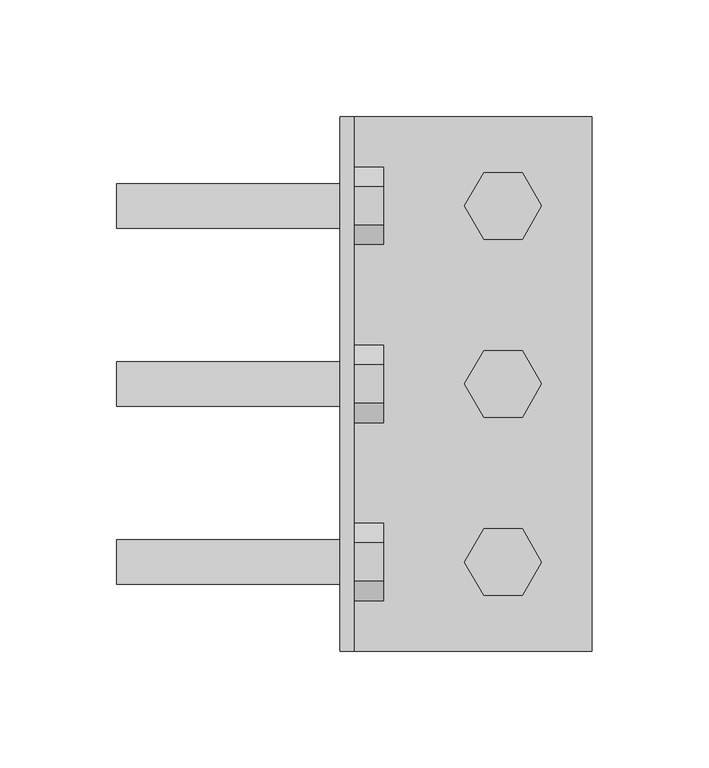
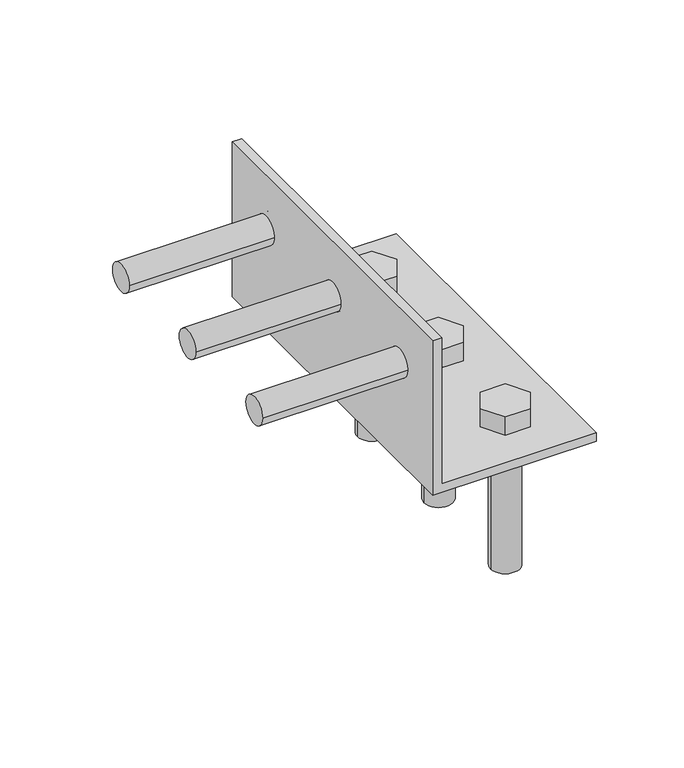
"""IFC4 building model written with IfcOpenShell, lengths in millimetres: fastener geometry, SIMPSON - HLPC/HLGPC Heavy Angles and Gussets : SIMPSON -HL49 - 9 X 4.25 - .75 Bolt - HDG."""

from ifc_helpers import new_model, si_unit, point, frame, frame_2d, origin, place, context, project, spatial, polyline, circle_curve, trimmed, segment, composite_curve, outline, extrude, source, transform, mapped, element, save
from ifc_brep_helpers import plane_surface, revolved_surface, advanced_brep


def fastener_80b0e17a(model_context):
    return source(origin(), model_context, "Body", "SolidModel", [
        extrude(outline(composite_curve([segment(trimmed(circle_curve(frame_2d((76.2, 69.85)), 9.525), [point((85.725, 69.85))], [point((66.675, 69.85))], False, "CARTESIAN"), True, "CONTINUOUS"), segment(trimmed(circle_curve(frame_2d((76.2, 69.85)), 9.525), [point((66.675, 69.85))], [point((85.725, 69.85))], False, "CARTESIAN"), True, "CONTINUOUS")], self_intersect=False)), frame((-95.5476562, 0.0, 0.0), z_axis=(1.0, 0.0, 0.0), x_axis=(0.0, 1.0, 0.0)), (0.0, 0.0, 1.0), 101.6),
        extrude(outline(polyline([(92.6977839, 69.85), (84.448892, 55.5625), (67.951108, 55.5625), (59.7022161, 69.85), (67.951108, 84.1375), (84.448892, 84.1375), (92.6977839, 69.85)])), frame((6.0523438, 0.0, 0.0), z_axis=(1.0, 0.0, 0.0), x_axis=(0.0, 1.0, 0.0)), (0.0, 0.0, 1.0), 12.7),
        extrude(outline(composite_curve([segment(trimmed(circle_curve(frame_2d((0.0, 69.85)), 9.525), [point((9.525, 69.85))], [point((-9.525, 69.85))], False, "CARTESIAN"), True, "CONTINUOUS"), segment(trimmed(circle_curve(frame_2d((0.0, 69.85)), 9.525), [point((-9.525, 69.85))], [point((9.525, 69.85))], False, "CARTESIAN"), True, "CONTINUOUS")], self_intersect=False)), frame((-95.5476562, 0.0, 0.0), z_axis=(1.0, 0.0, 0.0), x_axis=(0.0, 1.0, 0.0)), (0.0, 0.0, 1.0), 101.6),
        extrude(outline(polyline([(16.4977839, 69.85), (8.248892, 55.5625), (-8.248892, 55.5625), (-16.4977839, 69.85), (-8.248892, 84.1375), (8.248892, 84.1375), (16.4977839, 69.85)])), frame((6.0523438, 0.0, 0.0), z_axis=(1.0, 0.0, 0.0), x_axis=(0.0, 1.0, 0.0)), (0.0, 0.0, 1.0), 12.7),
        extrude(outline(composite_curve([segment(trimmed(circle_curve(frame_2d((-76.2, 69.85)), 9.525), [point((-66.675, 69.85))], [point((-85.725, 69.85))], False, "CARTESIAN"), True, "CONTINUOUS"), segment(trimmed(circle_curve(frame_2d((-76.2, 69.85)), 9.525), [point((-85.725, 69.85))], [point((-66.675, 69.85))], False, "CARTESIAN"), True, "CONTINUOUS")], self_intersect=False)), frame((-95.5476562, 0.0, 0.0), z_axis=(1.0, 0.0, 0.0), x_axis=(0.0, 1.0, 0.0)), (0.0, 0.0, 1.0), 101.6),
        extrude(outline(polyline([(-59.7022161, 69.85), (-67.951108, 55.5625), (-84.448892, 55.5625), (-92.6977839, 69.85), (-84.448892, 84.1375), (-67.951108, 84.1375), (-59.7022161, 69.85)])), frame((6.0523438, 0.0, 0.0), z_axis=(1.0, 0.0, 0.0), x_axis=(0.0, 1.0, 0.0)), (0.0, 0.0, 1.0), 12.7),
        extrude(outline(composite_curve([segment(trimmed(circle_curve(frame_2d((69.85, -76.2)), 9.525), [point((60.325, -76.2))], [point((79.375, -76.2))], False, "CARTESIAN"), True, "CONTINUOUS"), segment(trimmed(circle_curve(frame_2d((69.85, -76.2)), 9.525), [point((79.375, -76.2))], [point((60.325, -76.2))], False, "CARTESIAN"), True, "CONTINUOUS")], self_intersect=False)), frame((0.0, 0.0, -95.5476563), z_axis=(0.0, 0.0, 1.0), x_axis=(1.0, 0.0, 0.0)), (0.0, 0.0, 1.0), 101.6),
        extrude(outline(polyline([(53.3522161, -76.2), (61.601108, -61.9125), (78.098892, -61.9125), (86.3477839, -76.2), (78.098892, -90.4875), (61.601108, -90.4875), (53.3522161, -76.2)])), frame((0.0, 0.0, 6.0523437), z_axis=(0.0, 0.0, 1.0), x_axis=(1.0, 0.0, 0.0)), (0.0, 0.0, 1.0), 12.7),
        extrude(outline(composite_curve([segment(trimmed(circle_curve(frame_2d((69.85, 0.0)), 9.525), [point((60.325, 0.0))], [point((79.375, 0.0))], False, "CARTESIAN"), True, "CONTINUOUS"), segment(trimmed(circle_curve(frame_2d((69.85, 0.0)), 9.525), [point((79.375, 0.0))], [point((60.325, 0.0))], False, "CARTESIAN"), True, "CONTINUOUS")], self_intersect=False)), frame((0.0, 0.0, -95.5476563), z_axis=(0.0, 0.0, 1.0), x_axis=(1.0, 0.0, 0.0)), (0.0, 0.0, 1.0), 101.6),
        extrude(outline(polyline([(53.3522161, 0.0), (61.601108, 14.2875), (78.098892, 14.2875), (86.3477839, 0.0), (78.098892, -14.2875), (61.601108, -14.2875), (53.3522161, 0.0)])), frame((0.0, 0.0, 6.0523437), z_axis=(0.0, 0.0, 1.0), x_axis=(1.0, 0.0, 0.0)), (0.0, 0.0, 1.0), 12.7),
        extrude(outline(composite_curve([segment(trimmed(circle_curve(frame_2d((69.85, 76.2)), 9.525), [point((60.325, 76.2))], [point((79.375, 76.2))], False, "CARTESIAN"), True, "CONTINUOUS"), segment(trimmed(circle_curve(frame_2d((69.85, 76.2)), 9.525), [point((79.375, 76.2))], [point((60.325, 76.2))], False, "CARTESIAN"), True, "CONTINUOUS")], self_intersect=False)), frame((0.0, 0.0, -95.5476563), z_axis=(0.0, 0.0, 1.0), x_axis=(1.0, 0.0, 0.0)), (0.0, 0.0, 1.0), 101.6),
        extrude(outline(polyline([(53.3522161, 76.2), (61.601108, 90.4875), (78.098892, 90.4875), (86.3477839, 76.2), (78.098892, 61.9125), (61.601108, 61.9125), (53.3522161, 76.2)])), frame((0.0, 0.0, 6.0523437), z_axis=(0.0, 0.0, 1.0), x_axis=(1.0, 0.0, 0.0)), (0.0, 0.0, 1.0), 12.7),
        advanced_brep(
        [(6.0523438, -114.3, 107.95), (6.0523438, -114.3, 6.0523437), (6.0523438, 114.3, 6.0523437), (6.0523438, 114.3, 107.95), (6.0523438, 66.675, 69.85), (6.0523438, 85.725, 69.85), (6.0523438, -9.525, 69.85), (6.0523438, 9.525, 69.85), (6.0523438, -85.725, 69.85), (6.0523438, -66.675, 69.85), (0.0, 114.3, 107.95), (0.0, 114.3, 0.0), (0.0, -114.3, 0.0), (0.0, -114.3, 107.95), (0.0, 85.725, 69.85), (0.0, 66.675, 69.85), (0.0, 9.525, 69.85), (0.0, -9.525, 69.85), (0.0, -66.675, 69.85), (0.0, -85.725, 69.85), (107.95, 114.3, 6.0523437), (107.95, 114.3, 0.0), (107.95, -114.3, 0.0), (107.95, -114.3, 6.0523437), (79.375, 76.2, 6.0523437), (60.325, 76.2, 6.0523437), (79.375, 0.0, 6.0523437), (60.325, 0.0, 6.0523437), (79.375, -76.2, 6.0523437), (60.325, -76.2, 6.0523437), (60.325, 76.2, 0.0), (79.375, 76.2, 0.0), (60.325, 0.0, 0.0), (79.375, 0.0, 0.0), (60.325, -76.2, 0.0), (79.375, -76.2, 0.0)],
        [
            (0, 1),
            (1, 2),
            (2, 3),
            (3, 0),
            (4, 5, circle_curve(frame((6.0523438, 76.2, 69.85), z_axis=(-1.0, 0.0, 0.0), x_axis=(0.0, -1.0, 0.0)), 9.525)),
            (5, 4, circle_curve(frame((6.0523438, 76.2, 69.85), z_axis=(-1.0, 0.0, 0.0), x_axis=(0.0, -1.0, 0.0)), 9.525)),
            (6, 7, circle_curve(frame((6.0523438, 0.0, 69.85), z_axis=(-1.0, 0.0, 0.0), x_axis=(0.0, -1.0, 0.0)), 9.525)),
            (7, 6, circle_curve(frame((6.0523438, 0.0, 69.85), z_axis=(-1.0, 0.0, 0.0), x_axis=(0.0, -1.0, 0.0)), 9.525)),
            (8, 9, circle_curve(frame((6.0523438, -76.2, 69.85), z_axis=(-1.0, 0.0, 0.0), x_axis=(0.0, -1.0, 0.0)), 9.525)),
            (9, 8, circle_curve(frame((6.0523438, -76.2, 69.85), z_axis=(-1.0, 0.0, 0.0), x_axis=(0.0, -1.0, 0.0)), 9.525)),
            (10, 11),
            (11, 12),
            (12, 13),
            (13, 10),
            (14, 15, circle_curve(frame((0.0, 76.2, 69.85), z_axis=(1.0, 0.0, 0.0), x_axis=(0.0, -1.0, 0.0)), 9.525)),
            (15, 14, circle_curve(frame((0.0, 76.2, 69.85), z_axis=(1.0, 0.0, 0.0), x_axis=(0.0, -1.0, 0.0)), 9.525)),
            (16, 17, circle_curve(frame((0.0, 0.0, 69.85), z_axis=(1.0, 0.0, 0.0), x_axis=(0.0, -1.0, 0.0)), 9.525)),
            (17, 16, circle_curve(frame((0.0, 0.0, 69.85), z_axis=(1.0, 0.0, 0.0), x_axis=(0.0, -1.0, 0.0)), 9.525)),
            (18, 19, circle_curve(frame((0.0, -76.2, 69.85), z_axis=(1.0, 0.0, 0.0), x_axis=(0.0, -1.0, 0.0)), 9.525)),
            (19, 18, circle_curve(frame((0.0, -76.2, 69.85), z_axis=(1.0, 0.0, 0.0), x_axis=(0.0, -1.0, 0.0)), 9.525)),
            (3, 10),
            (13, 0),
            (2, 20),
            (20, 21),
            (21, 11),
            (12, 22),
            (22, 23),
            (23, 1),
            (23, 20),
            (24, 25, circle_curve(frame((69.85, 76.2, 6.0523437), z_axis=(0.0, 0.0, -1.0), x_axis=(1.0, 0.0, 0.0)), 9.525)),
            (25, 24, circle_curve(frame((69.85, 76.2, 6.0523437), z_axis=(0.0, 0.0, -1.0), x_axis=(1.0, 0.0, 0.0)), 9.525)),
            (26, 27, circle_curve(frame((69.85, 0.0, 6.0523437), z_axis=(0.0, 0.0, -1.0), x_axis=(1.0, 0.0, 0.0)), 9.525)),
            (27, 26, circle_curve(frame((69.85, 0.0, 6.0523437), z_axis=(0.0, 0.0, -1.0), x_axis=(1.0, 0.0, 0.0)), 9.525)),
            (28, 29, circle_curve(frame((69.85, -76.2, 6.0523437), z_axis=(0.0, 0.0, -1.0), x_axis=(1.0, 0.0, 0.0)), 9.525)),
            (29, 28, circle_curve(frame((69.85, -76.2, 6.0523437), z_axis=(0.0, 0.0, -1.0), x_axis=(1.0, 0.0, 0.0)), 9.525)),
            (21, 22),
            (30, 31, circle_curve(frame((69.85, 76.2, 0.0), z_axis=(0.0, 0.0, 1.0), x_axis=(1.0, 0.0, 0.0)), 9.525)),
            (31, 30, circle_curve(frame((69.85, 76.2, 0.0), z_axis=(0.0, 0.0, 1.0), x_axis=(1.0, 0.0, 0.0)), 9.525)),
            (32, 33, circle_curve(frame((69.85, 0.0, 0.0), z_axis=(0.0, 0.0, 1.0), x_axis=(1.0, 0.0, 0.0)), 9.525)),
            (33, 32, circle_curve(frame((69.85, 0.0, 0.0), z_axis=(0.0, 0.0, 1.0), x_axis=(1.0, 0.0, 0.0)), 9.525)),
            (34, 35, circle_curve(frame((69.85, -76.2, 0.0), z_axis=(0.0, 0.0, 1.0), x_axis=(1.0, 0.0, 0.0)), 9.525)),
            (35, 34, circle_curve(frame((69.85, -76.2, 0.0), z_axis=(0.0, 0.0, 1.0), x_axis=(1.0, 0.0, 0.0)), 9.525)),
            (25, 30),
            (31, 24),
            (27, 32),
            (33, 26),
            (29, 34),
            (35, 28),
            (5, 14),
            (15, 4),
            (7, 16),
            (17, 6),
            (9, 18),
            (19, 8),
        ],
        [
            plane_surface(frame((6.0523438, 114.3, 107.95), z_axis=(1.0, 0.0, 0.0), x_axis=(0.0, 1.0, 0.0))),
            plane_surface(frame((0.0, 114.3, 107.95), z_axis=(-1.0, 0.0, 0.0), x_axis=(0.0, -1.0, 0.0))),
            plane_surface(frame((6.0523438, -114.3, 107.95), z_axis=(0.0, 0.0, 1.0), x_axis=(-1.0, 0.0, 0.0))),
            plane_surface(frame((6.0523438, 114.3, 107.95), z_axis=(0.0, 1.0, 0.0), x_axis=(-1.0, 0.0, 0.0))),
            plane_surface(frame((6.0523438, -114.3, 6.0523437), z_axis=(0.0, -1.0, 0.0), x_axis=(-1.0, 0.0, 0.0))),
            plane_surface(frame((0.0, -114.3, 6.0523437), z_axis=(0.0, 0.0, 1.0), x_axis=(-1.0, 0.0, 0.0))),
            plane_surface(frame((0.0, -114.3, 0.0), z_axis=(0.0, 0.0, -1.0), x_axis=(1.0, 0.0, 0.0))),
            plane_surface(frame((107.95, 114.3, 6.0523437), z_axis=(1.0, 0.0, 0.0), x_axis=(0.0, 0.0, -1.0))),
            revolved_surface(polyline([(79.375, 76.2, 6.0523437), (79.375, 76.2, 0.0)]), (69.85, 76.2, 0.0), (0.0, 0.0, 1.0)),
            revolved_surface(polyline([(79.375, 0.0, 6.0523437), (79.375, 0.0, 0.0)]), (69.85, 0.0, 0.0), (0.0, 0.0, 1.0)),
            revolved_surface(polyline([(79.375, -76.2, 6.0523437), (79.375, -76.2, 0.0)]), (69.85, -76.2, 0.0), (0.0, 0.0, 1.0)),
            revolved_surface(polyline([(6.0523438, 66.675, 69.85), (0.0, 66.675, 69.85)]), (0.0, 76.2, 69.85), (1.0, 0.0, 0.0)),
            revolved_surface(polyline([(6.0523438, -9.525, 69.85), (0.0, -9.525, 69.85)]), (0.0, 0.0, 69.85), (1.0, 0.0, 0.0)),
            revolved_surface(polyline([(6.0523438, -85.72500000000001, 69.85), (0.0, -85.72500000000001, 69.85)]), (0.0, -76.2, 69.85), (1.0, 0.0, 0.0)),
        ],
        [
            (0, [[1, 2, 3, 4], [5, 6], [7, 8], [9, 10]]),
            (1, [[11, 12, 13, 14], [15, 16], [17, 18], [19, 20]]),
            (2, [[21, -14, 22, -4]]),
            (3, [[23, 24, 25, -11, -21, -3]]),
            (4, [[-22, -13, 26, 27, 28, -1]]),
            (5, [[-23, -2, -28, 29], [30, 31], [32, 33], [34, 35]]),
            (6, [[-26, -12, -25, 36], [37, 38], [39, 40], [41, 42]]),
            (7, [[-27, -36, -24, -29]]),
            (8, [[-31, 43, -38, 44]]),
            (8, [[-37, -43, -30, -44]]),
            (9, [[-33, 45, -40, 46]]),
            (9, [[-39, -45, -32, -46]]),
            (10, [[-35, 47, -42, 48]]),
            (10, [[-41, -47, -34, -48]]),
            (11, [[-6, 49, -16, 50]]),
            (11, [[-15, -49, -5, -50]]),
            (12, [[-8, 51, -18, 52]]),
            (12, [[-17, -51, -7, -52]]),
            (13, [[-10, 53, -20, 54]]),
            (13, [[-19, -53, -9, -54]]),
        ],
    ),
    ])


if __name__ == "__main__":
    model = new_model("IFC4")
    model_context = context("Model", 3, world=origin())
    ifc_project = project(units=[si_unit("LENGTHUNIT", "METRE", prefix="MILLI")], contexts=[model_context])
    site = spatial("IfcSite", under=ifc_project)
    building = spatial("IfcBuilding", under=site)
    placement = place(None, origin())
    fastener_shape = fastener_80b0e17a(model_context)
    element("IfcFastener", 1, ObjectType="SIMPSON - HLPC/HLGPC Heavy Angles and Gussets : SIMPSON -HL49 - 9 X 4.25 - .75 Bolt - HDG", at=placement, inside=building, context=model_context, shape_type="MappedRepresentation", body=[
        mapped(fastener_shape, transform((0.0, 0.0, 0.0), x_axis=(1.0, 0.0, 0.0), y_axis=(0.0, 1.0, 0.0), z_axis=(0.0, 0.0, 1.0))),
    ])
    save(model, "model.ifc")

# Revit data of these elements
# Type "SIMPSON - HLPC/HLGPC Heavy Angles and Gussets : SIMPSON -HL49 - 9 X 4.25 - .75 Bolt - HDG"
#   URL = "https://www.strongtie.com/classiccollection_architecturalproductsgroup/hlpc-hlgpc_productgroup_wcc/p/hlpc.hlgpc"
#   L = 0' - 9"
#   Hole Radius = 0' - 0 3/8"
#   D4 = 0' - 5"
#   D2 = 0' - 3"
#   D1 = 0' - 1 1/2"
#   D3 = 0' - 2 3/4"
#   Ga. = 0' - 0 61/256"
#   W1 & W2 = 0' - 4 1/4"
#   Default Elevation = 4' - 0"
#   Bolt Visibility - 3B = no
#   Bolt Visibility - 3A = yes
#   Bolt Visibility - 2B = no
#   Bolt Visibility - 2A = yes
#   Bolt Visibility - 1B = no
#   Bolt Visibility - 1A = yes
#   Bolt Visibility = yes
#   Bolt Size = element 1298415
# Element 1 (IfcFastener, "SIMPSON - HLPC/HLGPC Heavy Angles and Gussets : SIMPSON -HL49 - 9 X 4.25 - .75 Bolt - HDG")
#   Materials on its faces: "1\" GALV. LAG BOLT (LENGTH = 1/2\" SHY OF GLULAM DEPTH) -  (GALV. THRU BOLT IF PLATE ON OPP. SIDE OF STRUCT MEMBER)"
# Materials
#   "1\" GALV. LAG BOLT (LENGTH = 1/2\" SHY OF GLULAM DEPTH) -  (GALV. THRU BOLT IF PLATE ON OPP. SIDE OF STRUCT MEMBER)": class "Generic", colour RGB 120 120 120, transparency 0, Cost = 0
